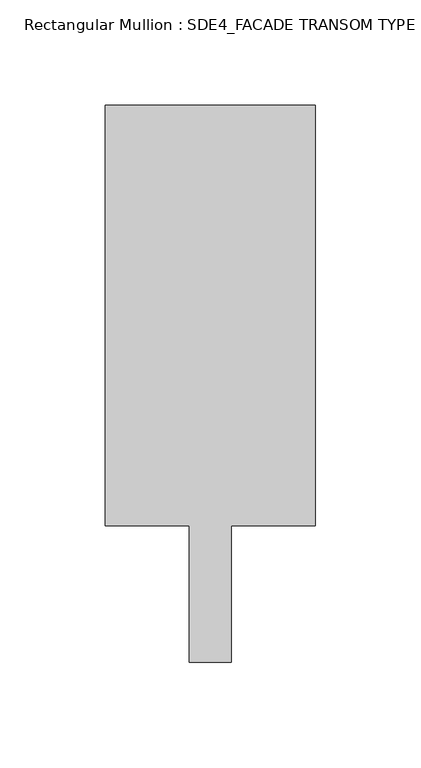
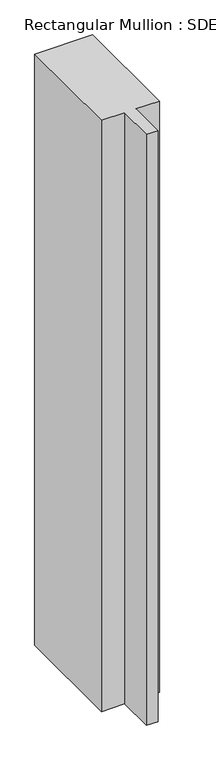
"""IFC4 building model written with IfcOpenShell, lengths in millimetres: member geometry, Rectangular Mullion : SDE4_FACADE TRANSOM TYPE 2."""

import ifcopenshell
import ifcopenshell.guid

model = None  # the IFC model being written
_history = None  # IfcOwnerHistory: only IFC2X3 demands one
_inside = {}  # id of a spatial element -> (the spatial element, [elements in it])
_under = {}  # id of a project, library or spatial element -> (it, [spatial elements below it])
_declared = {}  # id of a project -> (the project, [libraries it declares])
_typed = {}  # id of a type object -> (the type object, [elements of that type])
_made_of = {}  # id of a material, layer set ... -> (it, [elements and type objects made of it])


def new_model(schema):
    """Start an empty IFC model of exactly this schema.

    Asked for "IFC4X3", IfcOpenShell would pick the latest addendum, in which some entities
    have other attributes; the version numbers below select the first issue.
    IFC2X3 requires an IfcOwnerHistory on every rooted entity: one is made here for all.
    """
    global model, _history
    if schema == "IFC4X3":
        model = ifcopenshell.file(schema_version=(4, 3, 0, 0))
    else:
        model = ifcopenshell.file(schema=schema)
    _inside.clear()
    _under.clear()
    _declared.clear()
    _typed.clear()
    _made_of.clear()
    _history = None
    if model.schema == "IFC2X3":
        org = make("IfcOrganization", Name="unknown")
        user = make(
            "IfcPersonAndOrganization",
            ThePerson=make("IfcPerson", FamilyName="unknown"),
            TheOrganization=org,
        )
        app = make(
            "IfcApplication",
            ApplicationDeveloper=org,
            Version="unknown",
            ApplicationFullName="unknown",
            ApplicationIdentifier="unknown",
        )
        _history = make(
            "IfcOwnerHistory",
            OwningUser=user,
            OwningApplication=app,
            ChangeAction="ADDED",
            CreationDate=0,
        )
    return model


def make(cls, **values):
    """One entity of the class cls with the attributes given. An attribute that is None is left unset."""
    return model.create_entity(
        cls, **{name: value for name, value in values.items() if value is not None}
    )


def rooted(cls, **values):
    """An entity with a GlobalId (a new one), such as an element, a storey or a relation."""
    return make(cls, GlobalId=ifcopenshell.guid.new(), OwnerHistory=_history, **values)


def si_unit(unit_type, name, prefix=None):
    """IfcSIUnit, for example si_unit("LENGTHUNIT", "METRE", prefix="MILLI")."""
    return make("IfcSIUnit", UnitType=unit_type, Prefix=prefix, Name=name)


def assignment(units):
    """IfcUnitAssignment: the units of a project."""
    return None if units is None else make("IfcUnitAssignment", Units=units)


def point(xyz):
    """IfcCartesianPoint."""
    return None if xyz is None else make("IfcCartesianPoint", Coordinates=xyz)


def direction(xyz):
    """IfcDirection."""
    return None if xyz is None else make("IfcDirection", DirectionRatios=xyz)


def frame(location, z_axis=None, x_axis=None):
    """IfcAxis2Placement3D, a coordinate frame: its origin and axes. An axis left out is left unset."""
    return make(
        "IfcAxis2Placement3D",
        Location=point(location),
        Axis=direction(z_axis),
        RefDirection=direction(x_axis),
    )


def origin():
    """The frame at (0, 0, 0) with its axes left unset."""
    return frame((0.0, 0.0, 0.0))


def place(relative_to, where):
    """IfcLocalPlacement: puts the frame where relative to a parent placement (None: the world)."""
    return make(
        "IfcLocalPlacement", PlacementRelTo=relative_to, RelativePlacement=where
    )


def context(
    kind, dimensions, precision=None, world=None, true_north=None, identifier=None
):
    """IfcGeometricRepresentationContext, for example the 3D "Model" context."""
    return make(
        "IfcGeometricRepresentationContext",
        ContextIdentifier=identifier,
        ContextType=kind,
        CoordinateSpaceDimension=dimensions,
        Precision=precision,
        WorldCoordinateSystem=world,
        TrueNorth=true_north,
    )


def project(units=None, contexts=None):
    """IfcProject with its units and contexts."""
    return rooted(
        "IfcProject",
        Name="project",
        RepresentationContexts=contexts,
        UnitsInContext=assignment(units),
    )


def spatial(cls, under=None, at=None, **own):
    """A site, building, storey or space (cls), placed at a placement, below another one or the project."""
    s = rooted(cls, ObjectPlacement=at, **own)
    if under is not None:
        _under.setdefault(under.id(), (under, []))[1].append(s)
    return s


def polyline(points):
    """IfcPolyline through the points."""
    return make("IfcPolyline", Points=[point(p) for p in points])


def outline(outer, holes=None, kind="AREA"):
    """IfcArbitraryClosedProfileDef: a profile drawn as a closed curve; with holes, ...WithVoids."""
    if holes is None:
        return make("IfcArbitraryClosedProfileDef", ProfileType=kind, OuterCurve=outer)
    return make(
        "IfcArbitraryProfileDefWithVoids",
        ProfileType=kind,
        OuterCurve=outer,
        InnerCurves=holes,
    )


def extrude(swept, where, along, depth):
    """IfcExtrudedAreaSolid: the profile swept, set in the frame where, extruded along a direction by depth."""
    return make(
        "IfcExtrudedAreaSolid",
        SweptArea=swept,
        Position=where,
        ExtrudedDirection=direction(along),
        Depth=depth,
    )


def shape(context_of_items, identifier, shape_type, items):
    """IfcShapeRepresentation: the items that make up one representation, for example the "Body"."""
    return make(
        "IfcShapeRepresentation",
        ContextOfItems=context_of_items,
        RepresentationIdentifier=identifier,
        RepresentationType=shape_type,
        Items=items,
    )


def source(mapping_origin, context_of_items, identifier, shape_type, items):
    """IfcRepresentationMap: a shape defined once, which mapped items show again and again."""
    return make(
        "IfcRepresentationMap",
        MappingOrigin=mapping_origin,
        MappedRepresentation=shape(context_of_items, identifier, shape_type, items),
    )


def transform(
    local_origin,
    x_axis=None,
    y_axis=None,
    z_axis=None,
    scale=None,
    scale2=None,
    scale3=None,
    uniform=True,
):
    """IfcCartesianTransformationOperator3D, or its non-uniform kind. x_axis, y_axis, z_axis: its Axis1, 2, 3."""
    if uniform:
        return make(
            "IfcCartesianTransformationOperator3D",
            Axis1=direction(x_axis),
            Axis2=direction(y_axis),
            LocalOrigin=point(local_origin),
            Scale=scale,
            Axis3=direction(z_axis),
        )
    return make(
        "IfcCartesianTransformationOperator3DnonUniform",
        Axis1=direction(x_axis),
        Axis2=direction(y_axis),
        LocalOrigin=point(local_origin),
        Scale=scale,
        Axis3=direction(z_axis),
        Scale2=scale2,
        Scale3=scale3,
    )


def mapped(mapping_source, mapping_target):
    """IfcMappedItem: shows the shape of a source again, moved by a transform."""
    return make(
        "IfcMappedItem", MappingSource=mapping_source, MappingTarget=mapping_target
    )


def made_of(thing, what):
    """Note that an element or type object is made of a material, layer set ...; save() writes the relation."""
    if what is not None:
        _made_of.setdefault(what.id(), (what, []))[1].append(thing)
    return thing


def element(
    cls,
    number,
    at=None,
    inside=None,
    cuts=None,
    type_object=None,
    material=None,
    context=None,
    identifier="Body",
    shape_type=None,
    held_by="IfcProductDefinitionShape",
    body=None,
    shapes=None,
    **own,
):
    """One element of the class cls, such as IfcWall. Its Tag is "e" and its number.

    at: its placement. inside: the storey or other place that contains it. cuts: it is an
    opening in that element (IfcRelVoidsElement). A single representation is given by context,
    identifier, shape_type and body (its items); several are given by shapes. held_by: the class
    of the entity that holds the representations. save() writes the other relations.
    """
    e = rooted(cls, Tag="e%d" % number, ObjectPlacement=at, **own)
    if body is not None:
        shapes = [shape(context, identifier, shape_type, body)]
    if shapes is not None:
        e.Representation = make(held_by, Representations=shapes)
    if inside is not None:
        _inside.setdefault(inside.id(), (inside, []))[1].append(e)
    if cuts is not None:
        rooted(
            "IfcRelVoidsElement", RelatingBuildingElement=cuts, RelatedOpeningElement=e
        )
    if type_object is not None:
        _typed.setdefault(type_object.id(), (type_object, []))[1].append(e)
    return made_of(e, material)


def aggregate(whole, parts):
    """IfcRelAggregates: a whole, such as a stair, and the parts it consists of."""
    return rooted("IfcRelAggregates", RelatingObject=whole, RelatedObjects=parts)


def save(model, path):
    """Write the relations noted so far, then the file.

    IfcRelAggregates (storeys below a building ...), IfcRelContainedInSpatialStructure (elements
    in a storey), IfcRelDefinesByType, IfcRelAssociatesMaterial and IfcRelDeclares: one each for
    every whole, place, type object, material and project.
    """
    for whole, parts in _under.values():
        aggregate(whole, parts)
    for where, things in _inside.values():
        rooted(
            "IfcRelContainedInSpatialStructure",
            RelatedElements=things,
            RelatingStructure=where,
        )
    for kind, things in _typed.values():
        rooted("IfcRelDefinesByType", RelatedObjects=things, RelatingType=kind)
    for what, things in _made_of.values():
        rooted("IfcRelAssociatesMaterial", RelatedObjects=things, RelatingMaterial=what)
    for by, libraries in _declared.values():
        rooted("IfcRelDeclares", RelatingContext=by, RelatedDefinitions=libraries)
    model.write(path)


def rectangular_mullion_sde4_facade_transom_type_2_3e238be8(model_context):
    return source(origin(), model_context, "Body", "SweptSolid", [
        extrude(outline(polyline([(50.0, 132.5), (50.0, -67.5), (10.0, -67.5), (10.0, -132.5), (-10.0, -132.5), (-10.0, -67.5), (-50.0, -67.5), (-50.0, 132.5), (50.0, 132.5)])), frame((0.0, 0.0, -1079.375), z_axis=(0.0, 0.0, 1.0), x_axis=(1.0, 0.0, 0.0)), (0.0, 0.0, 1.0), 1079.375),
    ])


if __name__ == "__main__":
    model = new_model("IFC4")
    model_context = context("Model", 3, world=origin())
    ifc_project = project(units=[si_unit("LENGTHUNIT", "METRE", prefix="MILLI")], contexts=[model_context])
    site = spatial("IfcSite", under=ifc_project)
    building = spatial("IfcBuilding", under=site)
    placement = place(None, origin())
    rectangular_mullion_sde4_facade_transom_type_2_shape = rectangular_mullion_sde4_facade_transom_type_2_3e238be8(model_context)
    element("IfcMember", 1, ObjectType="Rectangular Mullion : SDE4_FACADE TRANSOM TYPE 2", at=placement, inside=building, context=model_context, shape_type="MappedRepresentation", body=[
        mapped(rectangular_mullion_sde4_facade_transom_type_2_shape, transform((0.0, 0.0, 0.0), x_axis=(1.0, 0.0, 0.0), y_axis=(0.0, 1.0, 0.0), z_axis=(0.0, 0.0, 1.0))),
    ])
    save(model, "model.ifc")

# Revit data of these elements
# Type "Rectangular Mullion : SDE4_FACADE TRANSOM TYPE 2"
#   built-in parameter 1007322 = 0.869423 (stored number, unit not read)
#   built-in parameter 1007321 = 0.164042 (stored number, unit not read)
#   built-in parameter 1007320 = 0.164042 (stored number, unit not read)
